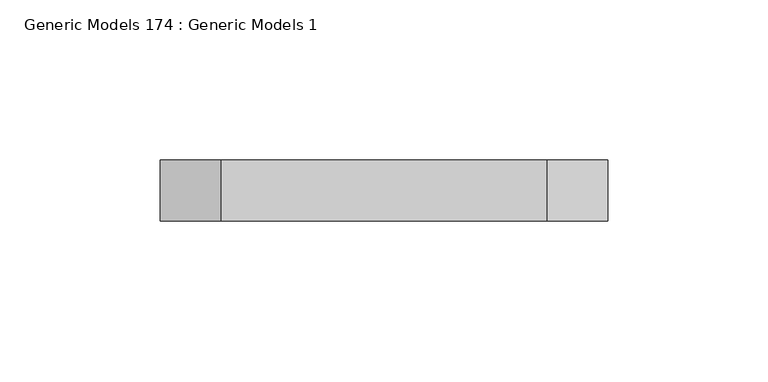
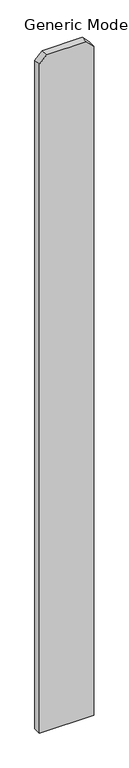
"""IFC4 building model written with IfcOpenShell, lengths in millimetres: proxy geometry, Generic Models 174 : Generic Models 1."""

from ifc_helpers import new_model, si_unit, frame, origin, place, context, project, spatial, polyline, outline, extrude, source, transform, mapped, element, save


def generic_models_174_generic_models_1_71a4a4c7(model_context):
    return source(origin(), model_context, "Body", "SweptSolid", [
        extrude(outline(polyline([(76.2, -248286.5875), (1885.95, -248286.5875), (1905.0, -248305.6375), (1905.0, -248407.2375), (1885.95, -248426.2875), (76.2, -248426.2875), (76.2, -248286.5875)])), frame((0.0, 547.6875, 0.0), z_axis=(0.0, 1.0, 0.0), x_axis=(0.0, 0.0, 1.0)), (0.0, 0.0, 1.0), 19.05),
    ])


if __name__ == "__main__":
    model = new_model("IFC4")
    model_context = context("Model", 3, world=origin())
    ifc_project = project(units=[si_unit("LENGTHUNIT", "METRE", prefix="MILLI")], contexts=[model_context])
    site = spatial("IfcSite", under=ifc_project)
    building = spatial("IfcBuilding", under=site)
    placement = place(None, origin())
    generic_models_174_generic_models_1_shape = generic_models_174_generic_models_1_71a4a4c7(model_context)
    element("IfcBuildingElementProxy", 1, Name="Generic Models 174 : Generic Models 1", ObjectType="Generic Models 174 : Generic Models 1", at=placement, inside=building, context=model_context, shape_type="MappedRepresentation", body=[
        mapped(generic_models_174_generic_models_1_shape, transform((0.0, 0.0, 0.0), x_axis=(1.0, 0.0, 0.0), y_axis=(0.0, 1.0, 0.0), z_axis=(0.0, 0.0, 1.0))),
    ])
    save(model, "model.ifc")

# Revit data of these elements
# Element 1 (IfcBuildingElementProxy, "Generic Models 174 : Generic Models 1")
#   Materials on its faces: "VERTICAL 1X6 CEDAR PLANKS W/ CLEAR WOOD SEALER"
# Materials
#   "VERTICAL 1X6 CEDAR PLANKS W/ CLEAR WOOD SEALER": class "Wood", colour RGB 234 198 147, transparency 0, Description = "Pinus Echinata", Cost = 0
